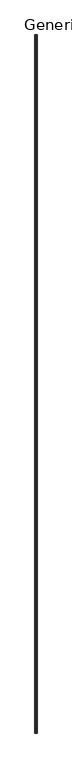
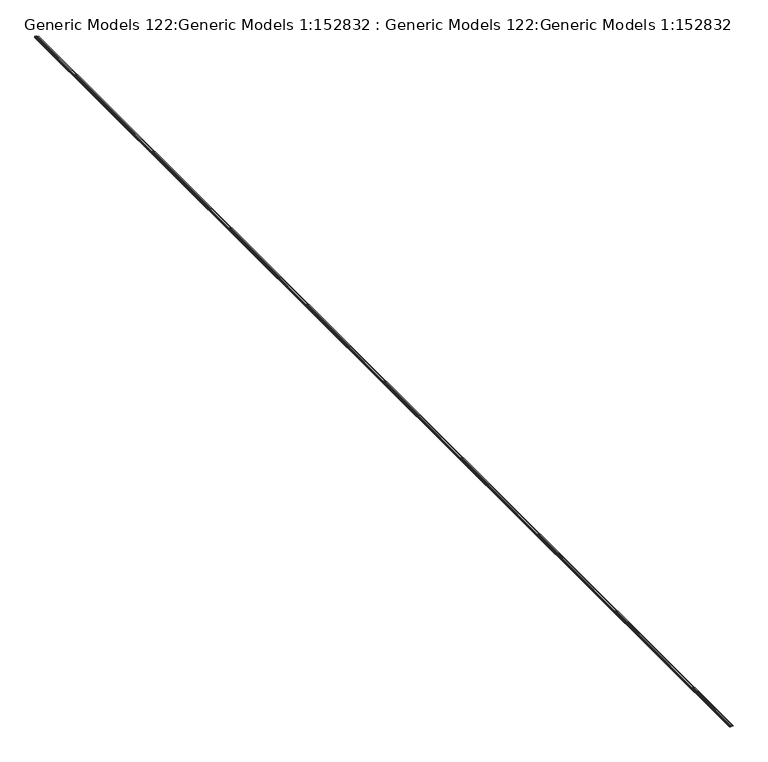
"""IFC4 building model written with IfcOpenShell, lengths in millimetres: proxy geometry, Generic Models 122:Generic Models 1:152832 : Generic Models 122:Generic Models 1:152832."""

from ifc_helpers import new_model, si_unit, frame, origin, place, context, project, spatial, polyline, outline, extrude, source, transform, mapped, element, save


def generic_models_122_generic_models_1_152832_generic_models_24b7bc9b(model_context):
    return source(origin(), model_context, "Body", "SweptSolid", [
        extrude(outline(polyline([(2896.6618287, -6668.3493913), (2896.6618287, -6688.0343913), (2898.8716287, -6688.0343913), (2898.8716287, -6687.1755504), (2919.1862074, -6687.1755504), (2919.1862074, -6688.4455504), (2900.1416287, -6688.4455504), (2900.1416287, -6689.3043913), (2895.3918287, -6689.3043913), (2895.3918287, -6667.0793913), (2906.8218287, -6667.0793913), (2906.8218287, -6654.3793913), (2895.3918287, -6654.3793913), (2895.3918287, -6630.6662074), (2896.6618287, -6630.6662074), (2896.6618287, -6653.1093913), (2908.0918287, -6653.1093913), (2908.0918287, -6668.3493913), (2896.6618287, -6668.3493913)])), frame((0.0, -6877.9974793, 0.0), z_axis=(0.0, 1.0, 0.0), x_axis=(0.0, 0.0, 1.0)), (0.0, 0.0, 1.0), 19050.0),
    ])


if __name__ == "__main__":
    model = new_model("IFC4")
    model_context = context("Model", 3, world=origin())
    ifc_project = project(units=[si_unit("LENGTHUNIT", "METRE", prefix="MILLI")], contexts=[model_context])
    site = spatial("IfcSite", under=ifc_project)
    building = spatial("IfcBuilding", under=site)
    placement = place(None, origin())
    generic_models_122_generic_models_1_152832_generic_models_shape = generic_models_122_generic_models_1_152832_generic_models_24b7bc9b(model_context)
    element("IfcBuildingElementProxy", 1, Name="Generic Models 122:Generic Models 1:152832 : Generic Models 122:Generic Models 1:152832", ObjectType="Generic Models 122:Generic Models 1:152832 : Generic Models 122:Generic Models 1:152832", at=placement, inside=building, context=model_context, shape_type="MappedRepresentation", body=[
        mapped(generic_models_122_generic_models_1_152832_generic_models_shape, transform((0.0, 0.0, 0.0), x_axis=(1.0, 0.0, 0.0), y_axis=(0.0, 1.0, 0.0), z_axis=(0.0, 0.0, 1.0))),
    ])
    save(model, "model.ifc")

# Revit data of these elements
# Type "Generic Models 122:Generic Models 1:152832 : Generic Models 122:Generic Models 1:152832"
#   NameOverride = "Generic Models 122:Generic Models 1:152832"
#   ObjectTypeOverride = "Generic Models 122:Generic Models 1"
#   Reference = "Generic Models 1"
#   Category = "Generic Models"
#   Tag = "152832"
# Element 1 (IfcBuildingElementProxy, "Generic Models 122:Generic Models 1:152832 : Generic Models 122:Generic Models 1:152832")
#   Materials on its faces: "_16 GA. COPPER SOFFIT DRIP SCREED 1359"
# Materials
#   "_16 GA. COPPER SOFFIT DRIP SCREED 1359": class "Unassigned", colour RGB 253 192 103, transparency 0
